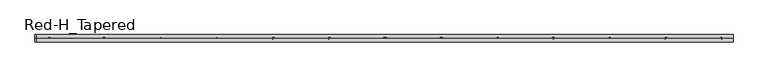
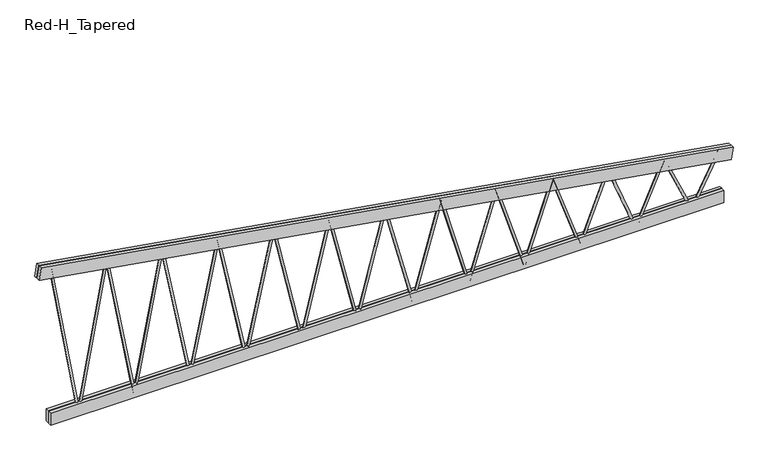
"""IFC4 building model written with IfcOpenShell, lengths in millimetres: beam geometry, Construction_Frames_RedBuilt_Openweb_Red-H_Tapered : Red-H_Tapered."""

from ifc_helpers import new_model, si_unit, point, frame, origin, origin_2d, place, context, project, spatial, polyline, circle_curve, trimmed, segment, composite_curve, outline, extrude, source, transform, mapped, element, save


def red_h_tapered_bf23eade(model_context):
    return source(origin(), model_context, "Body", "SweptSolid", [
        extrude(outline(composite_curve([segment(trimmed(circle_curve(origin_2d(), 12.7), [point((0.0, -12.7))], [point((0.0, 12.7000001))], False, "CARTESIAN"), True, "CONTINUOUS"), segment(trimmed(circle_curve(origin_2d(), 12.7), [point((0.0, 12.7000001))], [point((0.0, -12.7))], False, "CARTESIAN"), True, "CONTINUOUS")], self_intersect=False)), frame((-307.3140684, 0.0, -367.0101562), z_axis=(-0.23360956817291967, 0.0, 0.9723304837646828), x_axis=(0.0, -1.0, 0.0)), (0.0, 0.0, 1.0), 1315.502917),
        extrude(outline(composite_curve([segment(trimmed(circle_curve(origin_2d(), 12.7), [point((0.0, 12.7))], [point((0.0, -12.7000001))], False, "CARTESIAN"), True, "CONTINUOUS"), segment(trimmed(circle_curve(origin_2d(), 12.7), [point((0.0, -12.7000001))], [point((0.0, 12.7))], False, "CARTESIAN"), True, "CONTINUOUS")], self_intersect=False)), frame((-921.9422051, 0.0, -367.0101562), z_axis=(0.23360956817292067, 0.0, 0.9723304837646826), x_axis=(0.0, -1.0, 0.0)), (0.0, 0.0, 1.0), 1315.502917),
        extrude(outline(composite_curve([segment(trimmed(circle_curve(origin_2d(), 12.7), [point((0.0, -12.7))], [point((0.0, 12.6999999))], False, "CARTESIAN"), True, "CONTINUOUS"), segment(trimmed(circle_curve(origin_2d(), 12.7), [point((0.0, 12.6999999))], [point((0.0, -12.7))], False, "CARTESIAN"), True, "CONTINUOUS")], self_intersect=False)), frame((-921.9422051, 0.0, -367.0101562), z_axis=(-0.21761085323936008, 0.0, 0.9760356123382168), x_axis=(0.0, -1.0, 0.0)), (0.0, 0.0, 1.0), 1412.2184799),
        extrude(outline(composite_curve([segment(trimmed(circle_curve(origin_2d(), 12.7), [point((0.0, -12.7))], [point((0.0, 12.7))], False, "CARTESIAN"), True, "CONTINUOUS"), segment(trimmed(circle_curve(origin_2d(), 12.7), [point((0.0, 12.7))], [point((0.0, -12.7))], False, "CARTESIAN"), True, "CONTINUOUS")], self_intersect=False)), frame((-1536.5703419, 0.0, -367.0101562), z_axis=(0.21761085323936388, 0.0, 0.976035612338216), x_axis=(0.0, -1.0, 0.0)), (0.0, 0.0, 1.0), 1412.2184799),
        extrude(outline(composite_curve([segment(trimmed(circle_curve(origin_2d(), 12.7), [point((0.0, 12.6999999))], [point((0.0, -12.7000001))], False, "CARTESIAN"), True, "CONTINUOUS"), segment(trimmed(circle_curve(origin_2d(), 12.7), [point((0.0, -12.7000001))], [point((0.0, 12.6999999))], False, "CARTESIAN"), True, "CONTINUOUS")], self_intersect=False)), frame((-1536.5703419, 0.0, -367.0101562), z_axis=(-0.20361822241154776, 0.0, 0.9790503661722217), x_axis=(0.0, -1.0, 0.0)), (0.0, 0.0, 1.0), 1509.2660408),
        extrude(outline(composite_curve([segment(trimmed(circle_curve(origin_2d(), 12.7), [point((0.0, -12.6999999))], [point((0.0, 12.7000001))], False, "CARTESIAN"), True, "CONTINUOUS"), segment(trimmed(circle_curve(origin_2d(), 12.7), [point((0.0, 12.7000001))], [point((0.0, -12.6999999))], False, "CARTESIAN"), True, "CONTINUOUS")], self_intersect=False)), frame((-2151.1984787, 0.0, -367.0101562), z_axis=(0.2036182224115465, 0.0, 0.9790503661722221), x_axis=(0.0, -1.0, 0.0)), (0.0, 0.0, 1.0), 1509.2660408),
        extrude(outline(composite_curve([segment(trimmed(circle_curve(origin_2d(), 12.7), [point((0.0, 12.7000001))], [point((0.0, -12.7))], False, "CARTESIAN"), True, "CONTINUOUS"), segment(trimmed(circle_curve(origin_2d(), 12.7), [point((0.0, -12.7))], [point((0.0, 12.7000001))], False, "CARTESIAN"), True, "CONTINUOUS")], self_intersect=False)), frame((-2151.1984787, 0.0, -367.0101562), z_axis=(-0.19128398736508334, 0.0, 0.9815347350846605), x_axis=(0.0, -1.0, 0.0)), (0.0, 0.0, 1.0), 1606.5854367),
        extrude(outline(composite_curve([segment(trimmed(circle_curve(origin_2d(), 12.7), [point((0.0, -12.7000001))], [point((0.0, 12.7))], False, "CARTESIAN"), True, "CONTINUOUS"), segment(trimmed(circle_curve(origin_2d(), 12.7), [point((0.0, 12.7))], [point((0.0, -12.7000001))], False, "CARTESIAN"), True, "CONTINUOUS")], self_intersect=False)), frame((-2765.8266154, 0.0, -367.0101562), z_axis=(0.19128398736508884, 0.0, 0.9815347350846595), x_axis=(0.0, -1.0, 0.0)), (0.0, 0.0, 1.0), 1606.5854367),
        extrude(outline(composite_curve([segment(trimmed(circle_curve(origin_2d(), 12.7), [point((0.0, 12.7))], [point((0.0, -12.7))], False, "CARTESIAN"), True, "CONTINUOUS"), segment(trimmed(circle_curve(origin_2d(), 12.7), [point((0.0, -12.7))], [point((0.0, 12.7))], False, "CARTESIAN"), True, "CONTINUOUS")], self_intersect=False)), frame((-2765.8266154, 0.0, -367.0101562), z_axis=(-0.18033486353074976, 0.0, 0.9836052749936561), x_axis=(0.0, -1.0, 0.0)), (0.0, 0.0, 1.0), 1704.1300965),
        extrude(outline(composite_curve([segment(trimmed(circle_curve(origin_2d(), 12.7), [point((0.0, -12.7))], [point((0.0, 12.7))], False, "CARTESIAN"), True, "CONTINUOUS"), segment(trimmed(circle_curve(origin_2d(), 12.7), [point((0.0, 12.7))], [point((0.0, -12.7))], False, "CARTESIAN"), True, "CONTINUOUS")], self_intersect=False)), frame((-3380.4547522, 0.0, -367.0101562), z_axis=(0.18033486353074868, 0.0, 0.9836052749936564), x_axis=(0.0, -1.0, 0.0)), (0.0, 0.0, 1.0), 1704.1300965),
        extrude(outline(composite_curve([segment(trimmed(circle_curve(origin_2d(), 12.7), [point((0.0, 12.7))], [point((0.0, -12.7000001))], False, "CARTESIAN"), True, "CONTINUOUS"), segment(trimmed(circle_curve(origin_2d(), 12.7), [point((0.0, -12.7000001))], [point((0.0, 12.7))], False, "CARTESIAN"), True, "CONTINUOUS")], self_intersect=False)), frame((-3380.4547522, 0.0, -367.0101562), z_axis=(-0.17055347382480715, 0.0, 0.9853484219129246), x_axis=(0.0, -1.0, 0.0)), (0.0, 0.0, 1.0), 1801.8634361),
        extrude(outline(composite_curve([segment(trimmed(circle_curve(origin_2d(), 12.7), [point((0.0, 12.7))], [point((0.0, -12.6999999))], False, "CARTESIAN"), True, "CONTINUOUS"), segment(trimmed(circle_curve(origin_2d(), 12.7), [point((0.0, -12.6999999))], [point((0.0, 12.7))], False, "CARTESIAN"), True, "CONTINUOUS")], self_intersect=False)), frame((3380.4547522, 0.0, -367.0101562), z_axis=(0.4655570689406799, 0.0, 0.8850178617176961), x_axis=(0.0, -1.0, 0.0)), (0.0, 0.0, 1.0), 660.0996717),
        extrude(outline(composite_curve([segment(trimmed(circle_curve(origin_2d(), 12.7), [point((0.0, -12.7))], [point((0.0, 12.7))], False, "CARTESIAN"), True, "CONTINUOUS"), segment(trimmed(circle_curve(origin_2d(), 12.7), [point((0.0, 12.7))], [point((0.0, -12.7))], False, "CARTESIAN"), True, "CONTINUOUS")], self_intersect=False)), frame((3380.4547522, 0.0, -367.0101562), z_axis=(-0.41008911115791935, 0.0, 0.9120454598920538), x_axis=(0.0, -1.0, 0.0)), (0.0, 0.0, 1.0), 749.383634),
        extrude(outline(composite_curve([segment(trimmed(circle_curve(origin_2d(), 12.7), [point((0.0, 12.7000001))], [point((0.0, -12.7))], False, "CARTESIAN"), True, "CONTINUOUS"), segment(trimmed(circle_curve(origin_2d(), 12.7), [point((0.0, -12.7))], [point((0.0, 12.7000001))], False, "CARTESIAN"), True, "CONTINUOUS")], self_intersect=False)), frame((2765.8266154, 0.0, -367.0101562), z_axis=(0.4100891111579188, 0.0, 0.912045459892054), x_axis=(0.0, -1.0, 0.0)), (0.0, 0.0, 1.0), 749.383634),
        extrude(outline(composite_curve([segment(trimmed(circle_curve(origin_2d(), 12.7), [point((0.0, -12.7))], [point((0.0, 12.7))], False, "CARTESIAN"), True, "CONTINUOUS"), segment(trimmed(circle_curve(origin_2d(), 12.7), [point((0.0, 12.7))], [point((0.0, -12.7))], False, "CARTESIAN"), True, "CONTINUOUS")], self_intersect=False)), frame((2765.8266154, 0.0, -367.0101562), z_axis=(-0.3654540968364044, 0.0, 0.9308293630443165), x_axis=(0.0, -1.0, 0.0)), (0.0, 0.0, 1.0), 840.9101746),
        extrude(outline(composite_curve([segment(trimmed(circle_curve(origin_2d(), 12.7), [point((0.0, 12.7))], [point((0.0, -12.7))], False, "CARTESIAN"), True, "CONTINUOUS"), segment(trimmed(circle_curve(origin_2d(), 12.7), [point((0.0, -12.7))], [point((0.0, 12.7))], False, "CARTESIAN"), True, "CONTINUOUS")], self_intersect=False)), frame((2151.1984787, 0.0, -367.0101562), z_axis=(0.3654540968364036, 0.0, 0.9308293630443168), x_axis=(0.0, -1.0, 0.0)), (0.0, 0.0, 1.0), 840.9101746),
        extrude(outline(composite_curve([segment(trimmed(circle_curve(origin_2d(), 12.7), [point((0.0, -12.7))], [point((0.0, 12.7))], False, "CARTESIAN"), True, "CONTINUOUS"), segment(trimmed(circle_curve(origin_2d(), 12.7), [point((0.0, 12.7))], [point((0.0, -12.7))], False, "CARTESIAN"), True, "CONTINUOUS")], self_intersect=False)), frame((2151.1984787, 0.0, -367.0101562), z_axis=(-0.3290229141652683, 0.0, 0.9443219376643722), x_axis=(0.0, -1.0, 0.0)), (0.0, 0.0, 1.0), 934.0202617),
        extrude(outline(composite_curve([segment(trimmed(circle_curve(origin_2d(), 12.7), [point((0.0, 12.7))], [point((0.0, -12.7))], False, "CARTESIAN"), True, "CONTINUOUS"), segment(trimmed(circle_curve(origin_2d(), 12.7), [point((0.0, -12.7))], [point((0.0, 12.7))], False, "CARTESIAN"), True, "CONTINUOUS")], self_intersect=False)), frame((1536.5703419, 0.0, -367.0101562), z_axis=(0.3290229141652681, 0.0, 0.9443219376643723), x_axis=(0.0, -1.0, 0.0)), (0.0, 0.0, 1.0), 934.0202617),
        extrude(outline(composite_curve([segment(trimmed(circle_curve(origin_2d(), 12.7), [point((0.0, -12.7000001))], [point((0.0, 12.7))], False, "CARTESIAN"), True, "CONTINUOUS"), segment(trimmed(circle_curve(origin_2d(), 12.7), [point((0.0, 12.7))], [point((0.0, -12.7000001))], False, "CARTESIAN"), True, "CONTINUOUS")], self_intersect=False)), frame((1536.5703419, 0.0, -367.0101562), z_axis=(-0.2988611340441735, 0.0, 0.9542966114148319), x_axis=(0.0, -1.0, 0.0)), (0.0, 0.0, 1.0), 1028.2838194),
        extrude(outline(composite_curve([segment(trimmed(circle_curve(origin_2d(), 12.7), [point((0.0, 12.7000001))], [point((0.0, -12.6999999))], False, "CARTESIAN"), True, "CONTINUOUS"), segment(trimmed(circle_curve(origin_2d(), 12.7), [point((0.0, -12.6999999))], [point((0.0, 12.7000001))], False, "CARTESIAN"), True, "CONTINUOUS")], self_intersect=False)), frame((921.9422051, 0.0, -367.0101562), z_axis=(0.29886113404417736, 0.0, 0.9542966114148307), x_axis=(0.0, -1.0, 0.0)), (0.0, 0.0, 1.0), 1028.2838194),
        extrude(outline(composite_curve([segment(trimmed(circle_curve(origin_2d(), 12.7), [point((0.0, -12.7))], [point((0.0, 12.7000001))], False, "CARTESIAN"), True, "CONTINUOUS"), segment(trimmed(circle_curve(origin_2d(), 12.7), [point((0.0, 12.7000001))], [point((0.0, -12.7))], False, "CARTESIAN"), True, "CONTINUOUS")], self_intersect=False)), frame((921.9422051, 0.0, -367.0101562), z_axis=(-0.2735545562337163, 0.0, 0.9618564886529458), x_axis=(0.0, -1.0, 0.0)), (0.0, 0.0, 1.0), 1123.4105277),
        extrude(outline(composite_curve([segment(trimmed(circle_curve(origin_2d(), 12.7), [point((0.0, 12.7))], [point((0.0, -12.7))], False, "CARTESIAN"), True, "CONTINUOUS"), segment(trimmed(circle_curve(origin_2d(), 12.7), [point((0.0, -12.7))], [point((0.0, 12.7))], False, "CARTESIAN"), True, "CONTINUOUS")], self_intersect=False)), frame((307.3140684, 0.0, -367.0101562), z_axis=(0.2735545562337177, 0.0, 0.9618564886529455), x_axis=(0.0, -1.0, 0.0)), (0.0, 0.0, 1.0), 1123.4105277),
        extrude(outline(composite_curve([segment(trimmed(circle_curve(origin_2d(), 12.7), [point((0.0, -12.7))], [point((0.0, 12.7))], False, "CARTESIAN"), True, "CONTINUOUS"), segment(trimmed(circle_curve(origin_2d(), 12.7), [point((0.0, 12.7))], [point((0.0, -12.7))], False, "CARTESIAN"), True, "CONTINUOUS")], self_intersect=False)), frame((307.3140684, 0.0, -367.0101562), z_axis=(-0.252062402176264, 0.0, 0.967710982374971), x_axis=(0.0, -1.0, 0.0)), (0.0, 0.0, 1.0), 1219.1983641),
        extrude(outline(composite_curve([segment(trimmed(circle_curve(origin_2d(), 12.7), [point((0.0, 12.7))], [point((0.0, -12.7))], False, "CARTESIAN"), True, "CONTINUOUS"), segment(trimmed(circle_curve(origin_2d(), 12.7), [point((0.0, -12.7))], [point((0.0, 12.7))], False, "CARTESIAN"), True, "CONTINUOUS")], self_intersect=False)), frame((-307.3140684, 0.0, -367.0101562), z_axis=(0.25206240217622494, 0.0, 0.9677109823749812), x_axis=(0.0, -1.0, 0.0)), (0.0, 0.0, 1.0), 1219.1983641),
        extrude(outline(polyline([(-3713.1688206, -41.275), (-3713.1688206, -3.175), (3713.1688206, -3.175), (3713.1688206, -41.275), (-3713.1688206, -41.275)])), frame((0.0, 0.0, -386.0601562), z_axis=(0.0, 0.0, 1.0), x_axis=(1.0, 0.0, 0.0)), (0.0, 0.0, 1.0), 139.7),
        extrude(outline(polyline([(-3713.1688206, 3.175), (-3713.1688206, 41.275), (3713.1688206, 41.275), (3713.1688206, 3.175), (-3713.1688206, 3.175)])), frame((0.0, 0.0, -386.0601562), z_axis=(0.0, 0.0, 1.0), x_axis=(1.0, 0.0, 0.0)), (0.0, 0.0, 1.0), 139.7),
        extrude(outline(polyline([(0.0, -38.1), (0.0, 0.0), (7733.2170778, 0.0), (7733.2170778, -38.1), (0.0, -38.1)])), frame((-3837.5678872, -3.175, 1347.7753052), z_axis=(0.16320019046512393, 0.0, 0.9865929747530879), x_axis=(0.9865929747530879, 0.0, -0.16320019046512393)), (0.0, 0.0, 1.0), 139.7),
        extrude(outline(polyline([(0.0, -38.1), (0.0, 0.0), (7733.2170778, 0.0), (7733.2170778, -38.1), (0.0, -38.1)])), frame((-3837.5678872, 41.275, 1347.7753052), z_axis=(0.16320019046512393, 0.0, 0.9865929747530879), x_axis=(0.9865929747530879, 0.0, -0.16320019046512393)), (0.0, 0.0, 1.0), 139.7),
    ])


if __name__ == "__main__":
    model = new_model("IFC4")
    model_context = context("Model", 3, world=origin())
    ifc_project = project(units=[si_unit("LENGTHUNIT", "METRE", prefix="MILLI")], contexts=[model_context])
    site = spatial("IfcSite", under=ifc_project)
    building = spatial("IfcBuilding", under=site)
    placement = place(None, origin())
    red_h_tapered_shape = red_h_tapered_bf23eade(model_context)
    element("IfcBeam", 1, ObjectType="Construction_Frames_RedBuilt_Openweb_Red-H_Tapered : Red-H_Tapered", at=placement, inside=building, context=model_context, shape_type="MappedRepresentation", body=[
        mapped(red_h_tapered_shape, transform((0.0, 0.0, 0.0), x_axis=(1.0, 0.0, 0.0), y_axis=(0.0, 1.0, 0.0), z_axis=(0.0, 0.0, 1.0))),
    ])
    save(model, "model.ifc")

# Revit data of these elements
# Type "Construction_Frames_RedBuilt_Openweb_Red-H_Tapered : Red-H_Tapered"
#   Youtube clip = ""
#   Weight Net (Kg) = "0"
#   Webs = "Up to 2\" diameter tubular steel"
#   Uniformat II Description = ""
#   Uniformat II Code = ""
#   Uniclass 2015 Name = "Softwood trusses"
#   Uniclass 2015 Code = "Pr_20_85_90_81"
#   Uniclass 2.0 Description = "Structural Framing Systems"
#   Uniclass 2.0 Code = "SS-15-10-75"
#   Uniclass 1.4 Description = "Trusses"
#   Uniclass 1.4 Code = "L3523"
#   UNSPSC Code = "30103606"
#   Technical description = "http://www.redbuilt.com/reference/literature-and-other-resources"
#   Region South America = "None"
#   Region Oceania = "None"
#   Region North America = "US"
#   Region Middle East = "None"
#   Region Europe = "None"
#   Region Asia = "None"
#   Region Antarctica = "None"
#   Region Africa = "None"
#   QR code = "http://bimobject.com/redbuilt/product/redbuilt-0003"
#   Product url = "http://www.redbuilt.com/products/default.aspx?id=2"
#   Product group = "Wood Trusses"
#   Product family = "Construction"
#   Product data url = "https://bimobject.com/redbuilt/product/redbuilt-0003"
#   Product certification = ""
#   Product SKU = "redbuilt-0003"
#   Product Page URL = "http://www.redbuilt.com/commercial-systems/red-m-red-h-open-web-trusses"
#   Product Guid = "2c5793f2-6ffb-4665-b825-cf90c048e711"
#   Product Documentation Link = "http://www.redbuilt.com/documents/OW_Guide_2017_07_LowRes_wLinks.pdf"
#   OmniClass Description = "Wood Trusses"
#   OmniClass Code = "23-13 35 19 13 17"
#   NBS Reference Description = ""
#   NBS Reference Code = ""
#   Material secondary = "Steel"
#   Material main = "Wood"
#   Masterformat 2014 Description = "Metal-Web Wood Joists"
#   Masterformat 2014 Code = "06 17 36"
#   Manufacturer name = "RedBuilt"
#   Manufacturer country = "United States"
#   Installation instructions = "http://www.redbuilt.com/documents/Installation_Sheets_Open-Web.pdf"
#   IFC Classification = ""
#   EAN code = ""
#   Design country = "United States"
#   Product Information = "http://redbuilt.com/products/default.aspx?id=2"
#   Model = "Red-H-Tapered"
#   Manufacturer URL = "http://redbuilt.com/"
#   Manufacturer = "RedBuilt™"
#   Description = "Open Web Truss"
#   Date of publishing = "8/17/2010"
#   Contact us = "http://redbuilt.com/contact/"
#   Chords = "Double 1½\" x 5½\" MSR lumber"
#   COBIe Type Category = ""
#   Brand url = "http://www.redbuilt.com"
#   BIMobject main category code = "construction"
#   BIMobject main category = "Construction"
#   BIMobject category code = "construction-frames-trusses"
#   BIMobject category = "Frames & Trusses"
#   Web Radius = 0' - 0 1/2"
#   Web Layout Offset Start [instance default] = 0' - 5"
#   Web Layout Offset End [instance default] = 0' - 5"
#   Web Diameter = 0' - 1"
#   TotalLength [instance default] = 20' - 0"
#   Span Minimum = 4' - 0"
#   Span Maximum = 70' - 0"
#   Span Limit [instance default] = 20' - 0"
#   Nominal width = 0' - 0"
#   Nominal height = 0' - 0"
#   Inner Depth Top [instance default] = 0' - 2.76372"
#   Depth Start [instance default] = 6' - 0"
#   Top Chord Length [instance default] = 20' - 1.19701"
#   TC Extension Start Aux [instance default] = 0' - 0"
#   TC Extension End Aux [instance default] = 0' - 0"
#   T-B Chord Length Difference L [instance default] = 0' - 4"
#   T-B Chord Length Difference [instance default] = 0' - 4"
#   Height 2 [instance default] = 6' - 0"
#   Depth Minimum at Wall = 2' - 0"
#   Depth Maximum at Wall = 6' - 0"
#   Depth Lower End [instance default] = 2' - 0"
#   Depth Higher End [instance default] = 6' - 0"
#   Depth End [instance default] = 2' - 0"
#   Depth 2 [instance default] = 2' - 0"
#   Chord Width = 0' - 3 1/4"
#   Chord Thickness = 0' - 1 1/2"
#   Chord Depth = 0' - 5 1/2"
#   Offset Start [instance default] = 0' - 0"
#   TC Extension Start [instance default] = 0' - 0"
#   End Panel = 0' - 5"
#   Offset End [instance default] = 0' - 0"
#   TC Extension End [instance default] = 0' - 0"
#   Length [instance default] = 20' - 0"
#   Angle [instance default] = 5.71059°
#   Span Limit Warning [instance default] = no
#   Edition number = 1
#   Top Bearing Start [instance default] = yes
#   Top Bearing End [instance default] = yes
#   Bottom Bearing Start [instance default] = no
#   Bottom Bearing End [instance default] = no
#   8 Panels [instance default] = yes
#   16 Panels [instance default] = no
#   12 Panels [instance default] = no
#   Web Material = RedBuilt-Steel, Galvanized
#   Clip Material = RedBuilt-Steel, Galvanized
#   Chords Material = RedBuilt-MSR
#   URL = ""
#   Assembly Code = ""
# Element 1 (IfcBeam, "Construction_Frames_RedBuilt_Openweb_Red-H_Tapered : Red-H_Tapered")
#   TotalLength = 25' - 0.3755"
#   Span Limit = 25' - 0.3755"
#   Inner Depth Top = 0' - 2.78737"
#   Top Chord Length = 25' - 4.45737"
#   Depth 2 = 4' - 1 11/16"
#   Angle = 9.3927°
#   8 Panels = no
#   12 Panels = yes
#   Materials on its faces: "RedBuilt-Steel, Galvanized", "RedBuilt-MSR"
# Materials
#   "RedBuilt-Steel, Galvanized": class "Metal", colour RGB 164 172 176, transparency 0, Manufacturer = "RedBuilt. LLC", Comments = "Openweb Metal Web", URL = "http://www.redbuilt.com/", Description = "Galvanized steel", Cost = 0
#   "RedBuilt-MSR": class "Wood", colour RGB 213 182 136, transparency 0, Manufacturer = "RedBuilt, LLC", URL = "http://www.redbuilt.com/", Cost = 0
